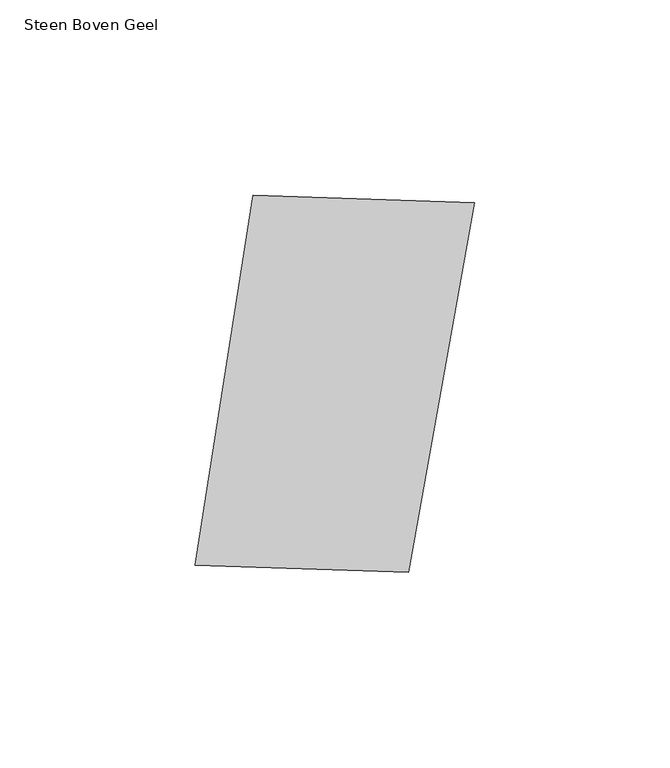
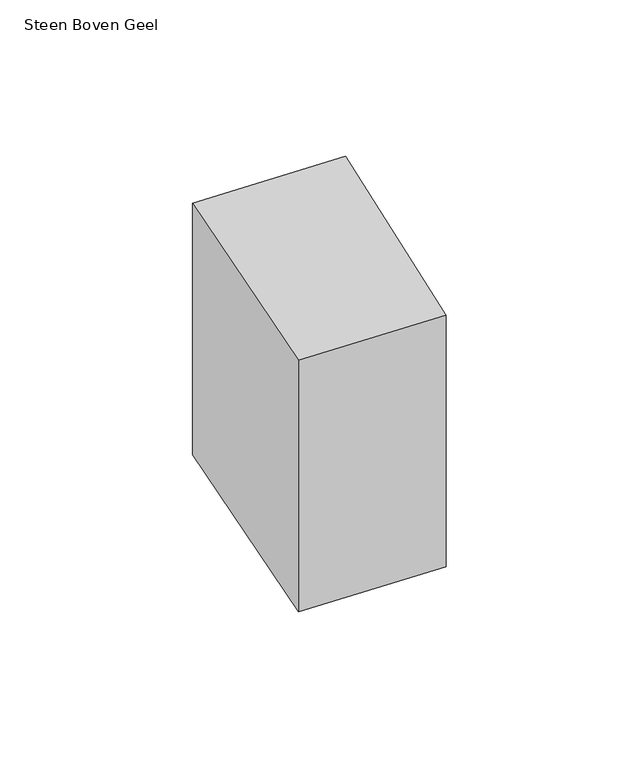
"""IFC4 building model written with IfcOpenShell, lengths in millimetres: proxy geometry, 00_GMA_steen_versie_4 : Steen Boven Geel."""

from ifc_helpers import new_model, si_unit, origin, origin_with_axes, place, context, project, spatial, polyline, outline, extrude, source, transform, mapped, element, save


def steen_boven_geel_ddefedde(model_context):
    return source(origin(), model_context, "Body", "SweptSolid", [
        extrude(outline(polyline([(109.4176759, 118.4962338), (92.5711073, 23.9486562), (38.0483358, 25.7540126), (52.7816307, 120.3588945), (109.4176759, 118.4962338)])), origin_with_axes(), (0.0, 0.0, 1.0), 100.0),
    ])


if __name__ == "__main__":
    model = new_model("IFC4")
    model_context = context("Model", 3, world=origin())
    ifc_project = project(units=[si_unit("LENGTHUNIT", "METRE", prefix="MILLI")], contexts=[model_context])
    site = spatial("IfcSite", under=ifc_project)
    building = spatial("IfcBuilding", under=site)
    placement = place(None, origin())
    steen_boven_geel_shape = steen_boven_geel_ddefedde(model_context)
    element("IfcBuildingElementProxy", 1, Name="00_GMA_steen_versie_4 : Steen Boven Geel", ObjectType="00_GMA_steen_versie_4 : Steen Boven Geel", at=placement, inside=building, context=model_context, shape_type="MappedRepresentation", body=[
        mapped(steen_boven_geel_shape, transform((0.0, 0.0, 0.0), x_axis=(1.0, 0.0, 0.0), y_axis=(0.0, 1.0, 0.0), z_axis=(0.0, 0.0, 1.0))),
    ])
    save(model, "model.ifc")

# Revit data of these elements
# Type "00_GMA_steen_versie_4 : Steen Boven Geel"
#   StootVoegHalfBoven [instance default] = 5 mm
#   StootVoegHalf [instance default] = 5 mm
#   StootVoegBreedteOnder = 10 mm
#   StootVoegBreedteBoven = 10 mm
#   Steendikte = 100 mm
#   LintVoegOnderHalf = 5 mm
#   LintVoegOnder = 10 mm
#   LintVoegBovenHalf = 0 mm
#   LintVoegBoven = 0 mm
#   materiaal = 21_steen_geel
#   MateriaalVoeg = none
#   Default Elevation = 0
# Element 1 (IfcBuildingElementProxy, "00_GMA_steen_versie_4 : Steen Boven Geel")
#   Materials on its faces: "21_steen_geel"
# Materials
#   "21_steen_geel": class "Unassigned", colour RGB 202 202 0, transparency 0, Cost = 0
